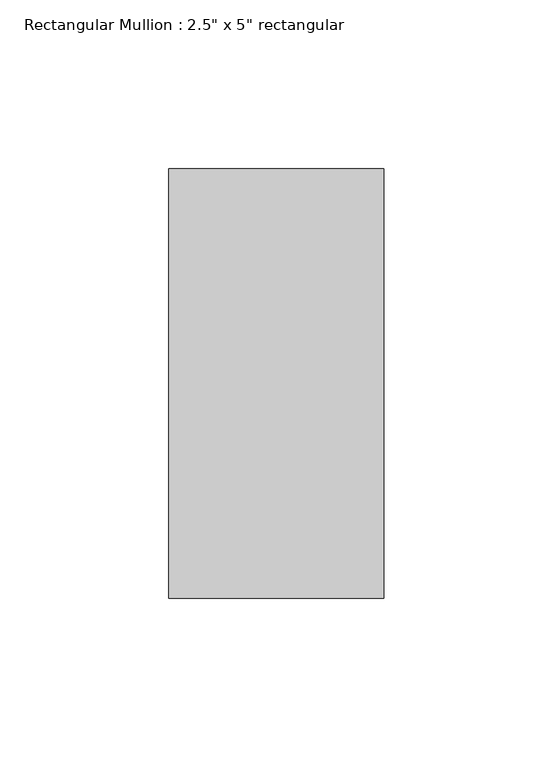
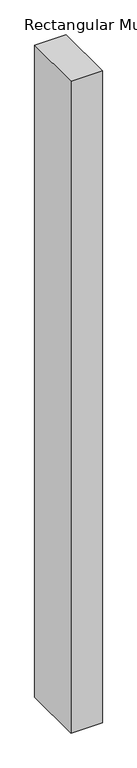
"""IFC4 building model written with IfcOpenShell, lengths in millimetres: member geometry."""

from ifc_helpers import new_model, si_unit, frame, origin, place, context, project, spatial, polyline, outline, extrude, source, transform, mapped, element, save


def member_0e9192ed(model_context):
    return source(origin(), model_context, "Body", "SweptSolid", [
        extrude(outline(polyline([(31.75, 63.5), (31.75, -63.5), (-31.75, -63.5), (-31.75, 63.5), (31.75, 63.5)])), frame((0.0, 0.0, -1394.8833336), z_axis=(0.0, 0.0, 1.0), x_axis=(1.0, 0.0, 0.0)), (0.0, 0.0, 1.0), 1394.8833336),
    ])


if __name__ == "__main__":
    model = new_model("IFC4")
    model_context = context("Model", 3, world=origin())
    ifc_project = project(units=[si_unit("LENGTHUNIT", "METRE", prefix="MILLI")], contexts=[model_context])
    site = spatial("IfcSite", under=ifc_project)
    building = spatial("IfcBuilding", under=site)
    placement = place(None, origin())
    member_shape = member_0e9192ed(model_context)
    element("IfcMember", 1, ObjectType="Rectangular Mullion : 2.5\" x 5\" rectangular", at=placement, inside=building, context=model_context, shape_type="MappedRepresentation", body=[
        mapped(member_shape, transform((0.0, 0.0, 0.0), x_axis=(1.0, 0.0, 0.0), y_axis=(0.0, 1.0, 0.0), z_axis=(0.0, 0.0, 1.0))),
    ])
    save(model, "model.ifc")

# Revit data of these elements
# Type "Rectangular Mullion : 2.5\" x 5\" rectangular"
#   built-in parameter 1007304 = 0.416667 (stored number, unit not read)
#   built-in parameter 1007301 = 0.104167 (stored number, unit not read)
#   built-in parameter 1007300 = 0.104167 (stored number, unit not read)
# Element 1 (IfcMember, "Rectangular Mullion : 2.5\" x 5\" rectangular")
#   Materials on its faces: "Aluminum"
# Materials
#   "Aluminum": class "Metal", colour RGB 247 247 247, transparency 0, Description = "Aluminum 6061", Cost = 0
